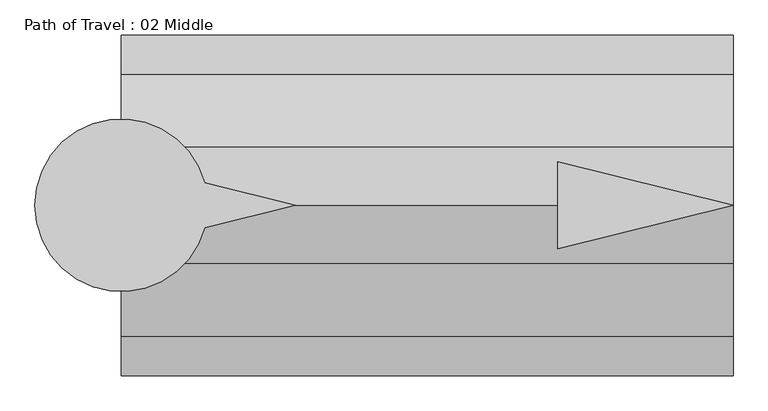
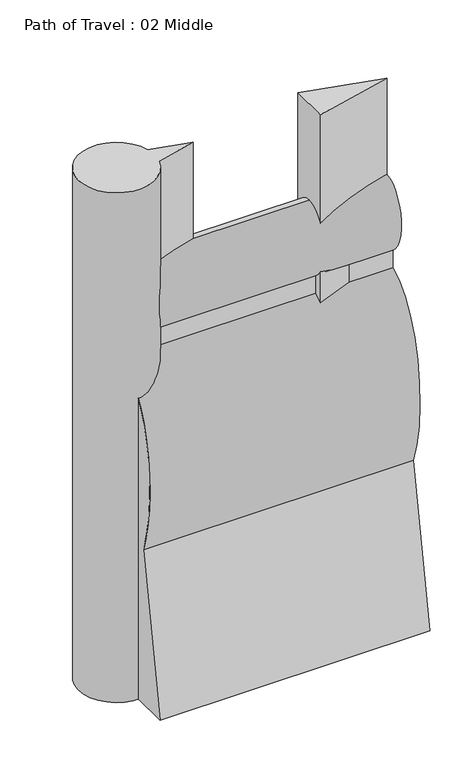
"""IFC4 building model written with IfcOpenShell, lengths in millimetres: proxy geometry, Path of Travel : 02 Middle."""

from ifc_helpers import new_model, si_unit, point, frame, frame_2d, origin, origin_with_axes, place, context, project, spatial, polyline, circle_curve, ellipse_curve, trimmed, segment, composite_curve, outline, extrude, source, transform, mapped, element, save
from ifc_brep_helpers import plane_surface, extruded_surface, advanced_brep


def path_of_travel_02_middle_6837fc71(model_context):
    return source(origin(), model_context, "Body", "SolidModel", [
        advanced_brep(
        [(227.5554837, 0.0, 1727.2), (227.5554837, 42.9018657, 1436.6534209), (227.5554837, 42.9018657, 1363.4763406), (227.5554837, 184.1186263, 643.4144547), (227.5554837, 297.5699544, 0.0), (227.5554837, 145.6574193, 0.0), (227.5554837, 0.0, 584.2), (227.5554837, -145.6574193, 0.0), (227.5554837, -297.5699544, 0.0), (227.5554837, -184.1186263, 643.4144547), (227.5554837, -42.9018657, 1363.4763406), (227.5554837, -42.9018657, 1436.6534209), (1296.3457734, 0.0, 1727.2), (1296.3457734, -42.9018657, 1436.6534209), (1296.3457734, -42.9018657, 1363.4763406), (1296.3457734, -184.1186263, 643.4144547), (1296.3457734, -297.5699544, 0.0), (1296.3457734, -145.6574193, 0.0), (1296.3457734, 0.0, 584.2), (1296.3457734, 145.6574193, 0.0), (1296.3457734, 297.5699544, 0.0), (1296.3457734, 184.1186263, 643.4144547), (1296.3457734, 42.9018657, 1363.4763406), (1296.3457734, 42.9018657, 1436.6534209)],
        [
            (0, 1, ellipse_curve(frame((227.5554837, 0.0, 1574.8), z_axis=(-1.0, 0.0, 0.0), x_axis=(0.0, 0.0, 1.0)), 152.4, 101.6)),
            (1, 2),
            (2, 3, ellipse_curve(frame((227.5554837, 0.0, 914.4), z_axis=(-1.0, 0.0, 0.0), x_axis=(0.0, 0.0, -1.0)), 457.2, 228.6)),
            (3, 4),
            (4, 5),
            (5, 6),
            (6, 7),
            (7, 8),
            (8, 9),
            (9, 10, ellipse_curve(frame((227.5554837, 0.0, 914.4), z_axis=(-1.0, 0.0, 0.0), x_axis=(0.0, 0.0, -1.0)), 457.2, 228.6)),
            (10, 11),
            (11, 0, ellipse_curve(frame((227.5554837, 0.0, 1574.8), z_axis=(-1.0, 0.0, 0.0), x_axis=(0.0, 0.0, 1.0)), 152.4, 101.6)),
            (12, 13, ellipse_curve(frame((1296.3457734, 0.0, 1574.8), z_axis=(1.0, 0.0, 0.0), x_axis=(0.0, 0.0, 1.0)), 152.4, 101.6)),
            (13, 14),
            (14, 15, ellipse_curve(frame((1296.3457734, 0.0, 914.4), z_axis=(1.0, 0.0, 0.0), x_axis=(0.0, 0.0, -1.0)), 457.2, 228.6)),
            (15, 16),
            (16, 17),
            (17, 18),
            (18, 19),
            (19, 20),
            (20, 21),
            (21, 22, ellipse_curve(frame((1296.3457734, 0.0, 914.4), z_axis=(1.0, 0.0, 0.0), x_axis=(0.0, 0.0, -1.0)), 457.2, 228.6)),
            (22, 23),
            (23, 12, ellipse_curve(frame((1296.3457734, 0.0, 1574.8), z_axis=(1.0, 0.0, 0.0), x_axis=(0.0, 0.0, 1.0)), 152.4, 101.6)),
            (0, 12),
            (23, 1),
            (22, 2),
            (21, 3),
            (20, 4),
            (19, 5),
            (18, 6),
            (17, 7),
            (16, 8),
            (15, 9),
            (14, 10),
            (13, 11),
        ],
        [
            plane_surface(frame((227.5554837, 0.0, 0.0), z_axis=(-1.0, 0.0, 0.0), x_axis=(0.0, 0.0, 1.0))),
            plane_surface(frame((1296.3457734, 0.0, 0.0), z_axis=(1.0, 0.0, 0.0), x_axis=(0.0, 0.0, 1.0))),
            extruded_surface(trimmed(ellipse_curve(frame((1296.3457734, 0.0, 1574.8), z_axis=(-1.0, 0.0, 0.0), x_axis=(0.0, 0.0, 1.0)), 152.4, 101.6), [point((1296.3457734, 0.0, 1727.2))], [point((1296.3457734, 42.9018657, 1436.6534209))], True, "CARTESIAN"), (-1068.7902897000001, 0.0, 0.0), 1068.7902897000001),
            plane_surface(frame((227.5554837, 42.9018657, 1436.6534209), z_axis=(0.0, 1.0, 0.0), x_axis=(1.0, 0.0, 0.0))),
            extruded_surface(trimmed(ellipse_curve(frame((1296.3457734, 0.0, 914.4), z_axis=(-1.0, 0.0, 0.0), x_axis=(0.0, 0.0, -1.0)), 457.2, 228.6), [point((1296.3457734, 42.9018657, 1363.4763406))], [point((1296.3457734, 184.1186263, 643.4144547))], True, "CARTESIAN"), (-1068.7902897000001, 0.0, 0.0), 1068.7902897000001),
            plane_surface(frame((227.5554837, 184.1186263, 643.4144547), z_axis=(0.0, 0.9848077530122078, 0.1736481776669322), x_axis=(1.0, 0.0, 0.0))),
            plane_surface(frame((227.5554837, 297.5699544, 0.0), z_axis=(0.0, 0.0, -1.0), x_axis=(1.0, 0.0, 0.0))),
            plane_surface(frame((227.5554837, 145.6574193, 0.0), z_axis=(0.0, -0.9702957262760199, -0.2419218955995739), x_axis=(1.0, 0.0, 0.0))),
            plane_surface(frame((227.5554837, 0.0, 584.2), z_axis=(0.0, 0.9702957262759961, -0.24192189559966923), x_axis=(1.0, 0.0, 0.0))),
            plane_surface(frame((227.5554837, -145.6574193, 0.0), z_axis=(0.0, 0.0, -1.0), x_axis=(1.0, 0.0, 0.0))),
            plane_surface(frame((227.5554837, -297.5699544, 0.0), z_axis=(0.0, -0.984807753012208, 0.17364817766693066), x_axis=(1.0, 0.0, 0.0))),
            extruded_surface(trimmed(ellipse_curve(frame((1296.3457734, 0.0, 914.4), z_axis=(-1.0, 0.0, 0.0), x_axis=(0.0, 0.0, -1.0)), 457.2, 228.6), [point((1296.3457734, -184.1186263, 643.4144547))], [point((1296.3457734, -42.9018657, 1363.4763406))], True, "CARTESIAN"), (-1068.7902897000001, 0.0, 0.0), 1068.7902897000001),
            plane_surface(frame((227.5554837, -42.9018657, 1363.4763406), z_axis=(0.0, -1.0, 0.0), x_axis=(1.0, 0.0, 0.0))),
            extruded_surface(trimmed(ellipse_curve(frame((1296.3457734, 0.0, 1574.8), z_axis=(-1.0, 0.0, 0.0), x_axis=(0.0, 0.0, 1.0)), 152.4, 101.6), [point((1296.3457734, -42.9018657, 1436.6534209))], [point((1296.3457734, 0.0, 1727.2))], True, "CARTESIAN"), (-1068.7902897000001, 0.0, 0.0), 1068.7902897000001),
        ],
        [
            (0, [[1, 2, 3, 4, 5, 6, 7, 8, 9, 10, 11, 12]]),
            (1, [[13, 14, 15, 16, 17, 18, 19, 20, 21, 22, 23, 24]]),
            (2, [[-1, 25, -24, 26]]),
            (3, [[-2, -26, -23, 27]]),
            (4, [[-3, -27, -22, 28]]),
            (5, [[-4, -28, -21, 29]]),
            (6, [[-5, -29, -20, 30]]),
            (7, [[-6, -30, -19, 31]]),
            (8, [[-7, -31, -18, 32]]),
            (9, [[-8, -32, -17, 33]]),
            (10, [[-9, -33, -16, 34]]),
            (11, [[-10, -34, -15, 35]]),
            (12, [[-11, -35, -14, 36]]),
            (13, [[-12, -36, -13, -25]]),
        ],
    ),
        extrude(outline(polyline([(990.3406268, 76.2006338), (1296.3457734, 0.0), (990.3406268, -76.2006338), (990.3406268, 76.2006338)])), origin_with_axes(), (0.0, 0.0, 1.0), 2129.5973753),
        extrude(outline(composite_curve([segment(polyline([(372.7837828, 39.4440225), (531.182385, 0.0), (372.7837828, -39.4440225)]), True, "CONTINUOUS"), segment(trimmed(circle_curve(frame_2d((227.2200886, 0.0)), 150.8131956), [point((372.7837828, -39.4440225))], [point((372.7837828, 39.4440225))], False, "CARTESIAN"), True, "CONTINUOUS")], self_intersect=False)), origin_with_axes(), (0.0, 0.0, 1.0), 2129.5973753),
    ])


if __name__ == "__main__":
    model = new_model("IFC4")
    model_context = context("Model", 3, world=origin())
    ifc_project = project(units=[si_unit("LENGTHUNIT", "METRE", prefix="MILLI")], contexts=[model_context])
    site = spatial("IfcSite", under=ifc_project)
    building = spatial("IfcBuilding", under=site)
    placement = place(None, origin())
    path_of_travel_02_middle_shape = path_of_travel_02_middle_6837fc71(model_context)
    element("IfcBuildingElementProxy", 1, Name="Path of Travel : 02 Middle", ObjectType="Path of Travel : 02 Middle", at=placement, inside=building, context=model_context, shape_type="MappedRepresentation", body=[
        mapped(path_of_travel_02_middle_shape, transform((0.0, 0.0, 0.0), x_axis=(1.0, 0.0, 0.0), y_axis=(0.0, 1.0, 0.0), z_axis=(0.0, 0.0, 1.0))),
    ])
    save(model, "model.ifc")

# Revit data of these elements
# Type "Path of Travel : 02 Middle"
#   Path of Egress [instance default] = 4' - 0"
#   built-in parameter 1001306 [instance default] = 4 (stored number, unit not read)
#   Dot at Start = no
#   Arrow in Middle = yes
#   Arrow at End = no
#   Egress Path = none
# Element 1 (IfcBuildingElementProxy, "Path of Travel : 02 Middle")
#   Path of Egress = 3' - 6.07836"
#   built-in parameter 1001306 = 3.50653 (stored number, unit not read)
